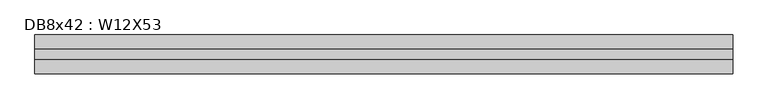
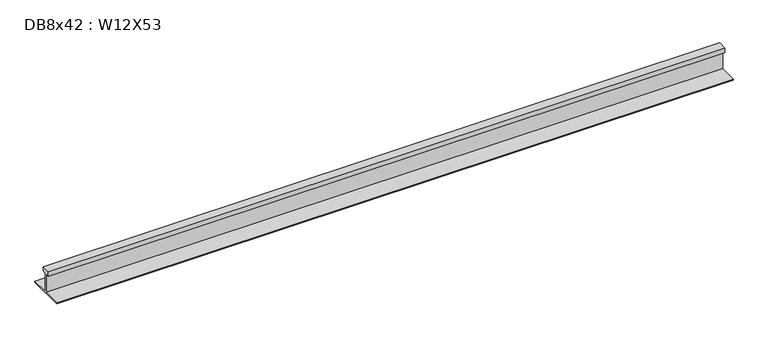
"""IFC4 building model written with IfcOpenShell, lengths in millimetres: beam geometry, DB8x42 : W12X53."""

from ifc_helpers import new_model, si_unit, frame, origin, place, context, project, spatial, polyline, outline, extrude, source, transform, mapped, element, save


def db8x42_w12x53_34813089(model_context):
    return source(origin(), model_context, "Body", "SweptSolid", [
        extrude(outline(polyline([(38.1, 144.3355), (38.1, 106.2355), (4.7625, 106.2355), (4.7625, -49.53), (152.4, -49.53), (152.4, -59.182), (-152.4, -59.182), (-152.4, -49.53), (-4.7625, -49.53), (-4.7625, 106.2355), (-38.1, 106.2355), (-38.1, 144.3355), (38.1, 144.3355)])), frame((-2743.2, 0.0, 0.0), z_axis=(1.0, 0.0, 0.0), x_axis=(0.0, 1.0, 0.0)), (0.0, 0.0, 1.0), 5486.4),
    ])


if __name__ == "__main__":
    model = new_model("IFC4")
    model_context = context("Model", 3, world=origin())
    ifc_project = project(units=[si_unit("LENGTHUNIT", "METRE", prefix="MILLI")], contexts=[model_context])
    site = spatial("IfcSite", under=ifc_project)
    building = spatial("IfcBuilding", under=site)
    placement = place(None, origin())
    db8x42_w12x53_shape = db8x42_w12x53_34813089(model_context)
    element("IfcBeam", 1, ObjectType="DB8x42 : W12X53", at=placement, inside=building, context=model_context, shape_type="MappedRepresentation", body=[
        mapped(db8x42_w12x53_shape, transform((0.0, 0.0, 0.0), x_axis=(1.0, 0.0, 0.0), y_axis=(0.0, 1.0, 0.0), z_axis=(0.0, 0.0, 1.0))),
    ])
    save(model, "model.ifc")

# Revit data of these elements
# Type "DB8x42 : W12X53"
#   Assembly Code = "B10"
#   W = 53
#   Length [instance default] = 5' - 0"
#   bf = 0' - 10"
#   d = 1' - 0.1"
#   k = 0' - 1 3/8"
#   k2 = 0' - 0.8"
#   tf = 0' - 0.575"
#   tw = 0' - 0.345"
#   A = 0.108333 SF
#   Structural Material [instance default] = Steel ASTM A992
# Element 1 (IfcBeam, "DB8x42 : W12X53")
#   Materials on its faces: "Steel ASTM A992"
# Materials
#   "Steel ASTM A992": class "Metal", colour RGB 199 199 199, transparency 0, Description = "Structural steel 50ksi", Cost = 0
